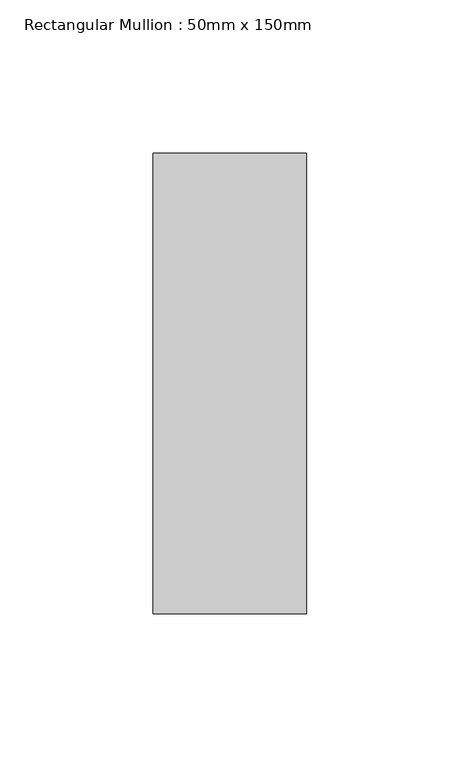
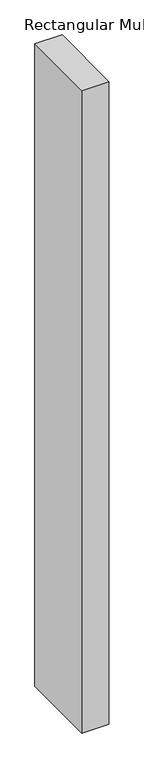
"""IFC4 building model written with IfcOpenShell, lengths in millimetres: member geometry, Rectangular Mullion : 50mm x 150mm."""

import ifcopenshell
import ifcopenshell.guid

model = None  # the IFC model being written
_history = None  # IfcOwnerHistory: only IFC2X3 demands one
_inside = {}  # id of a spatial element -> (the spatial element, [elements in it])
_under = {}  # id of a project, library or spatial element -> (it, [spatial elements below it])
_declared = {}  # id of a project -> (the project, [libraries it declares])
_typed = {}  # id of a type object -> (the type object, [elements of that type])
_made_of = {}  # id of a material, layer set ... -> (it, [elements and type objects made of it])


def new_model(schema):
    """Start an empty IFC model of exactly this schema.

    Asked for "IFC4X3", IfcOpenShell would pick the latest addendum, in which some entities
    have other attributes; the version numbers below select the first issue.
    IFC2X3 requires an IfcOwnerHistory on every rooted entity: one is made here for all.
    """
    global model, _history
    if schema == "IFC4X3":
        model = ifcopenshell.file(schema_version=(4, 3, 0, 0))
    else:
        model = ifcopenshell.file(schema=schema)
    _inside.clear()
    _under.clear()
    _declared.clear()
    _typed.clear()
    _made_of.clear()
    _history = None
    if model.schema == "IFC2X3":
        org = make("IfcOrganization", Name="unknown")
        user = make(
            "IfcPersonAndOrganization",
            ThePerson=make("IfcPerson", FamilyName="unknown"),
            TheOrganization=org,
        )
        app = make(
            "IfcApplication",
            ApplicationDeveloper=org,
            Version="unknown",
            ApplicationFullName="unknown",
            ApplicationIdentifier="unknown",
        )
        _history = make(
            "IfcOwnerHistory",
            OwningUser=user,
            OwningApplication=app,
            ChangeAction="ADDED",
            CreationDate=0,
        )
    return model


def make(cls, **values):
    """One entity of the class cls with the attributes given. An attribute that is None is left unset."""
    return model.create_entity(
        cls, **{name: value for name, value in values.items() if value is not None}
    )


def rooted(cls, **values):
    """An entity with a GlobalId (a new one), such as an element, a storey or a relation."""
    return make(cls, GlobalId=ifcopenshell.guid.new(), OwnerHistory=_history, **values)


def si_unit(unit_type, name, prefix=None):
    """IfcSIUnit, for example si_unit("LENGTHUNIT", "METRE", prefix="MILLI")."""
    return make("IfcSIUnit", UnitType=unit_type, Prefix=prefix, Name=name)


def assignment(units):
    """IfcUnitAssignment: the units of a project."""
    return None if units is None else make("IfcUnitAssignment", Units=units)


def point(xyz):
    """IfcCartesianPoint."""
    return None if xyz is None else make("IfcCartesianPoint", Coordinates=xyz)


def direction(xyz):
    """IfcDirection."""
    return None if xyz is None else make("IfcDirection", DirectionRatios=xyz)


def frame(location, z_axis=None, x_axis=None):
    """IfcAxis2Placement3D, a coordinate frame: its origin and axes. An axis left out is left unset."""
    return make(
        "IfcAxis2Placement3D",
        Location=point(location),
        Axis=direction(z_axis),
        RefDirection=direction(x_axis),
    )


def origin():
    """The frame at (0, 0, 0) with its axes left unset."""
    return frame((0.0, 0.0, 0.0))


def place(relative_to, where):
    """IfcLocalPlacement: puts the frame where relative to a parent placement (None: the world)."""
    return make(
        "IfcLocalPlacement", PlacementRelTo=relative_to, RelativePlacement=where
    )


def context(
    kind, dimensions, precision=None, world=None, true_north=None, identifier=None
):
    """IfcGeometricRepresentationContext, for example the 3D "Model" context."""
    return make(
        "IfcGeometricRepresentationContext",
        ContextIdentifier=identifier,
        ContextType=kind,
        CoordinateSpaceDimension=dimensions,
        Precision=precision,
        WorldCoordinateSystem=world,
        TrueNorth=true_north,
    )


def project(units=None, contexts=None):
    """IfcProject with its units and contexts."""
    return rooted(
        "IfcProject",
        Name="project",
        RepresentationContexts=contexts,
        UnitsInContext=assignment(units),
    )


def spatial(cls, under=None, at=None, **own):
    """A site, building, storey or space (cls), placed at a placement, below another one or the project."""
    s = rooted(cls, ObjectPlacement=at, **own)
    if under is not None:
        _under.setdefault(under.id(), (under, []))[1].append(s)
    return s


def polyline(points):
    """IfcPolyline through the points."""
    return make("IfcPolyline", Points=[point(p) for p in points])


def outline(outer, holes=None, kind="AREA"):
    """IfcArbitraryClosedProfileDef: a profile drawn as a closed curve; with holes, ...WithVoids."""
    if holes is None:
        return make("IfcArbitraryClosedProfileDef", ProfileType=kind, OuterCurve=outer)
    return make(
        "IfcArbitraryProfileDefWithVoids",
        ProfileType=kind,
        OuterCurve=outer,
        InnerCurves=holes,
    )


def extrude(swept, where, along, depth):
    """IfcExtrudedAreaSolid: the profile swept, set in the frame where, extruded along a direction by depth."""
    return make(
        "IfcExtrudedAreaSolid",
        SweptArea=swept,
        Position=where,
        ExtrudedDirection=direction(along),
        Depth=depth,
    )


def shape(context_of_items, identifier, shape_type, items):
    """IfcShapeRepresentation: the items that make up one representation, for example the "Body"."""
    return make(
        "IfcShapeRepresentation",
        ContextOfItems=context_of_items,
        RepresentationIdentifier=identifier,
        RepresentationType=shape_type,
        Items=items,
    )


def source(mapping_origin, context_of_items, identifier, shape_type, items):
    """IfcRepresentationMap: a shape defined once, which mapped items show again and again."""
    return make(
        "IfcRepresentationMap",
        MappingOrigin=mapping_origin,
        MappedRepresentation=shape(context_of_items, identifier, shape_type, items),
    )


def transform(
    local_origin,
    x_axis=None,
    y_axis=None,
    z_axis=None,
    scale=None,
    scale2=None,
    scale3=None,
    uniform=True,
):
    """IfcCartesianTransformationOperator3D, or its non-uniform kind. x_axis, y_axis, z_axis: its Axis1, 2, 3."""
    if uniform:
        return make(
            "IfcCartesianTransformationOperator3D",
            Axis1=direction(x_axis),
            Axis2=direction(y_axis),
            LocalOrigin=point(local_origin),
            Scale=scale,
            Axis3=direction(z_axis),
        )
    return make(
        "IfcCartesianTransformationOperator3DnonUniform",
        Axis1=direction(x_axis),
        Axis2=direction(y_axis),
        LocalOrigin=point(local_origin),
        Scale=scale,
        Axis3=direction(z_axis),
        Scale2=scale2,
        Scale3=scale3,
    )


def mapped(mapping_source, mapping_target):
    """IfcMappedItem: shows the shape of a source again, moved by a transform."""
    return make(
        "IfcMappedItem", MappingSource=mapping_source, MappingTarget=mapping_target
    )


def made_of(thing, what):
    """Note that an element or type object is made of a material, layer set ...; save() writes the relation."""
    if what is not None:
        _made_of.setdefault(what.id(), (what, []))[1].append(thing)
    return thing


def element(
    cls,
    number,
    at=None,
    inside=None,
    cuts=None,
    type_object=None,
    material=None,
    context=None,
    identifier="Body",
    shape_type=None,
    held_by="IfcProductDefinitionShape",
    body=None,
    shapes=None,
    **own,
):
    """One element of the class cls, such as IfcWall. Its Tag is "e" and its number.

    at: its placement. inside: the storey or other place that contains it. cuts: it is an
    opening in that element (IfcRelVoidsElement). A single representation is given by context,
    identifier, shape_type and body (its items); several are given by shapes. held_by: the class
    of the entity that holds the representations. save() writes the other relations.
    """
    e = rooted(cls, Tag="e%d" % number, ObjectPlacement=at, **own)
    if body is not None:
        shapes = [shape(context, identifier, shape_type, body)]
    if shapes is not None:
        e.Representation = make(held_by, Representations=shapes)
    if inside is not None:
        _inside.setdefault(inside.id(), (inside, []))[1].append(e)
    if cuts is not None:
        rooted(
            "IfcRelVoidsElement", RelatingBuildingElement=cuts, RelatedOpeningElement=e
        )
    if type_object is not None:
        _typed.setdefault(type_object.id(), (type_object, []))[1].append(e)
    return made_of(e, material)


def aggregate(whole, parts):
    """IfcRelAggregates: a whole, such as a stair, and the parts it consists of."""
    return rooted("IfcRelAggregates", RelatingObject=whole, RelatedObjects=parts)


def save(model, path):
    """Write the relations noted so far, then the file.

    IfcRelAggregates (storeys below a building ...), IfcRelContainedInSpatialStructure (elements
    in a storey), IfcRelDefinesByType, IfcRelAssociatesMaterial and IfcRelDeclares: one each for
    every whole, place, type object, material and project.
    """
    for whole, parts in _under.values():
        aggregate(whole, parts)
    for where, things in _inside.values():
        rooted(
            "IfcRelContainedInSpatialStructure",
            RelatedElements=things,
            RelatingStructure=where,
        )
    for kind, things in _typed.values():
        rooted("IfcRelDefinesByType", RelatedObjects=things, RelatingType=kind)
    for what, things in _made_of.values():
        rooted("IfcRelAssociatesMaterial", RelatedObjects=things, RelatingMaterial=what)
    for by, libraries in _declared.values():
        rooted("IfcRelDeclares", RelatingContext=by, RelatedDefinitions=libraries)
    model.write(path)


def rectangular_mullion_50mm_x_150mm_302a0cfa(model_context):
    return source(origin(), model_context, "Body", "SweptSolid", [
        extrude(outline(polyline([(0.0, 75.0), (0.0, -75.0), (-50.0, -75.0), (-50.0, 75.0), (0.0, 75.0)])), frame((0.0, 0.0, -1253.5714288), z_axis=(0.0, 0.0, 1.0), x_axis=(1.0, 0.0, 0.0)), (0.0, 0.0, 1.0), 1253.5714288),
    ])


if __name__ == "__main__":
    model = new_model("IFC4")
    model_context = context("Model", 3, world=origin())
    ifc_project = project(units=[si_unit("LENGTHUNIT", "METRE", prefix="MILLI")], contexts=[model_context])
    site = spatial("IfcSite", under=ifc_project)
    building = spatial("IfcBuilding", under=site)
    placement = place(None, origin())
    rectangular_mullion_50mm_x_150mm_shape = rectangular_mullion_50mm_x_150mm_302a0cfa(model_context)
    element("IfcMember", 1, ObjectType="Rectangular Mullion : 50mm x 150mm", at=placement, inside=building, context=model_context, shape_type="MappedRepresentation", body=[
        mapped(rectangular_mullion_50mm_x_150mm_shape, transform((0.0, 0.0, 0.0), x_axis=(1.0, 0.0, 0.0), y_axis=(0.0, 1.0, 0.0), z_axis=(0.0, 0.0, 1.0))),
    ])
    save(model, "model.ifc")

# Revit data of these elements
# Type "Rectangular Mullion : 50mm x 150mm"
#   built-in parameter 1007304 = 0.492126 (stored number, unit not read)
#   built-in parameter 1007301 = 0.082021 (stored number, unit not read)
#   built-in parameter 1007300 = 0.082021 (stored number, unit not read)
# Element 1 (IfcMember, "Rectangular Mullion : 50mm x 150mm")
#   Materials on its faces: "Aluminum"
# Materials
#   "Aluminum": class "Metal", colour RGB 247 247 247, transparency 0, Description = "Aluminum 6061", Cost = 0
